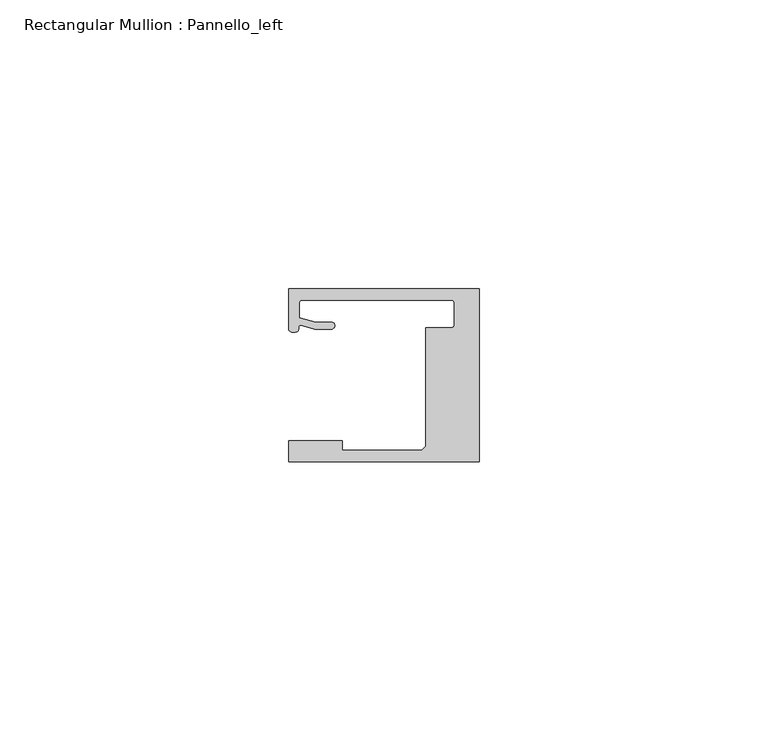
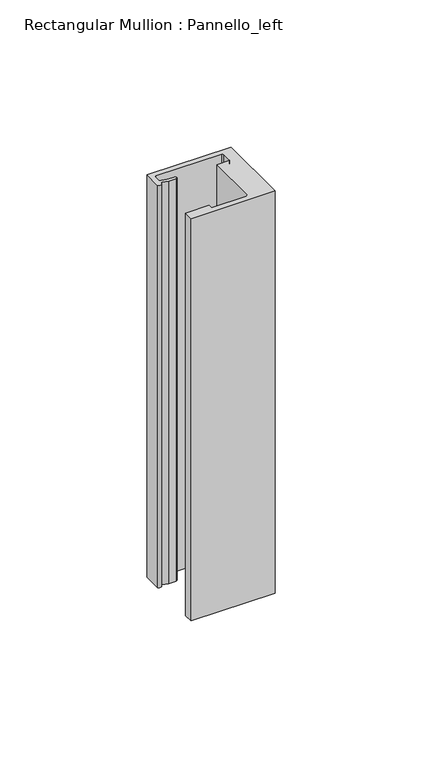
"""IFC4 building model written with IfcOpenShell, lengths in millimetres: member geometry, Rectangular Mullion : Pannello_left."""

from ifc_helpers import new_model, si_unit, frame, origin, place, context, project, spatial, polyline, circle_curve, source, transform, mapped, element, save
from ifc_brep_helpers import plane_surface, cylinder_surface, revolved_surface, extruded_surface, spline_curve, advanced_brep


def rectangular_mullion_pannello_left_600754f7(model_context):
    return source(origin(), model_context, "Body", "AdvancedBrep", [
        advanced_brep(
        [(-33.0, -15.0, 0.0), (0.0, -15.0, 0.0), (0.0, 15.0, 0.0), (-33.0000135, 15.0, 0.0), (-33.0000135, 8.0000472, 0.0), (-30.9223017, 8.6490241, 0.0), (-28.4999305, 7.9999523, 0.0), (-25.59998, 7.9999523, 0.0), (-25.59998, 9.1999523, 0.0), (-28.3419477, 9.1999523, 0.0), (-31.19998, 9.9657591, 0.0), (-31.19998, 12.50001, 0.0), (-30.69998, 13.00001, 0.0), (-4.7999726, 13.00001, 0.0), (-4.2999726, 12.50001, 0.0), (-4.2999726, 8.7500595, 0.0), (-4.7999726, 8.2500595, 0.0), (-9.2999726, 8.2500595, 0.0), (-9.2999726, -12.2999849, 0.0), (-10.0000103, -13.0000004, 0.0), (-23.700041, -13.0000004, 0.0), (-23.700041, -11.3000004, 0.0), (-33.0, -11.3000004, 0.0), (-33.0, -15.0, -166.9999865), (-33.0, -11.3000004, -166.9999865), (-23.700041, -11.3000004, -166.9999865), (-23.700041, -13.0000004, -166.9999865), (-10.0000103, -13.0000004, -166.9999865), (-9.2999726, -12.2999849, -166.9999865), (-9.2999726, 8.2500595, -166.9999865), (-4.7999726, 8.2500595, -166.9999865), (-4.2999726, 8.7500595, -166.9999865), (-4.2999726, 12.50001, -166.9999865), (-4.7999726, 13.00001, -166.9999865), (-30.69998, 13.00001, -166.9999865), (-31.19998, 12.50001, -166.9999865), (-31.19998, 9.9657591, -166.9999865), (-28.3419477, 9.1999523, -166.9999865), (-25.59998, 9.1999523, -166.9999865), (-25.59998, 7.9999523, -166.9999865), (-28.4999305, 7.9999523, -166.9999865), (-30.9223017, 8.6490241, -166.9999865), (-33.0000135, 8.0000472, -166.9999865), (-33.0000135, 15.0, -166.9999865), (0.0, 15.0, -166.9999865), (0.0, -15.0, -166.9999865)],
        [
            (0, 1),
            (1, 2),
            (2, 3),
            (3, 4),
            (4, 5, spline_curve(3, [(-33.0000135, 8.0000472, 0.0), (-33.0000135, 7.457047519, 0.0), (-32.262327879, 7.456527435, 0.0), (-31.357433266, 7.563996614, 0.0), (-31.305645054, 7.690065204, 0.0), (-31.298563602, 8.366228555, 0.0), (-31.312054066, 8.717747958, 0.0), (-30.9223017, 8.6490241, 0.0)], [4, 2, 2, 4], [0.0, 0.0027053965905959043, 0.0058611956533709, 0.007702013405570312])),
            (5, 6),
            (6, 7),
            (7, 8, circle_curve(frame((-25.59998, 8.5999523, 0.0), z_axis=(0.0, 0.0, 1.0), x_axis=(0.0, 1.0, 0.0)), 0.6)),
            (8, 9),
            (9, 10),
            (10, 11),
            (11, 12, circle_curve(frame((-30.69998, 12.50001, 0.0), z_axis=(0.0, 0.0, -1.0), x_axis=(0.0, 1.0, 0.0)), 0.5)),
            (12, 13),
            (13, 14, circle_curve(frame((-4.7999726, 12.50001, 0.0), z_axis=(0.0, 0.0, -1.0), x_axis=(1.0, 0.0, 0.0)), 0.5)),
            (14, 15),
            (15, 16, circle_curve(frame((-4.7999726, 8.7500595, 0.0), z_axis=(0.0, 0.0, -1.0), x_axis=(0.0, -1.0, 0.0)), 0.5)),
            (16, 17),
            (17, 18),
            (18, 19),
            (19, 20),
            (20, 21),
            (21, 22),
            (22, 0),
            (23, 24),
            (24, 25),
            (25, 26),
            (26, 27),
            (27, 28),
            (28, 29),
            (29, 30),
            (30, 31, circle_curve(frame((-4.7999726, 8.7500595, -166.9999865), z_axis=(0.0, 0.0, 1.0), x_axis=(0.0, -1.0, 0.0)), 0.5)),
            (31, 32),
            (32, 33, circle_curve(frame((-4.7999726, 12.50001, -166.9999865), z_axis=(0.0, 0.0, 1.0), x_axis=(1.0, 0.0, 0.0)), 0.5)),
            (33, 34),
            (34, 35, circle_curve(frame((-30.69998, 12.50001, -166.9999865), z_axis=(0.0, 0.0, 1.0), x_axis=(0.0, 1.0, 0.0)), 0.5)),
            (35, 36),
            (36, 37),
            (37, 38),
            (38, 39, circle_curve(frame((-25.59998, 8.5999523, -166.9999865), z_axis=(0.0, 0.0, -1.0), x_axis=(0.0, 1.0, 0.0)), 0.6)),
            (39, 40),
            (40, 41),
            (41, 42, spline_curve(3, [(-30.9223017, 8.6490241, -166.9999865), (-31.312054066, 8.717747958, -166.9999865), (-31.298563602, 8.366228555, -166.9999865), (-31.305645054, 7.690065204, -166.9999865), (-31.357433266, 7.563996614, -166.9999865), (-32.262327879, 7.456527435, -166.9999865), (-33.0000135, 7.457047519, -166.9999865), (-33.0000135, 8.0000472, -166.9999865)], [4, 2, 2, 4], [0.0, 0.001840817752199412, 0.004996616814974408, 0.007702013405570312])),
            (42, 43),
            (43, 44),
            (44, 45),
            (45, 23),
            (0, 23),
            (45, 1),
            (44, 2),
            (43, 3),
            (42, 4),
            (41, 5),
            (40, 6),
            (39, 7),
            (38, 8),
            (37, 9),
            (36, 10),
            (35, 11),
            (34, 12),
            (33, 13),
            (32, 14),
            (31, 15),
            (30, 16),
            (29, 17),
            (28, 18),
            (27, 19),
            (26, 20),
            (25, 21),
            (24, 22),
        ],
        [
            plane_surface(frame((0.0, -36.2491502, 0.0), z_axis=(0.0, 0.0, 1.0), x_axis=(-1.0, 0.0, 0.0))),
            plane_surface(frame((0.0, -36.2491502, -166.9999865), z_axis=(0.0, 0.0, -1.0), x_axis=(-1.0, 0.0, 0.0))),
            plane_surface(frame((-33.0, -15.0, 0.0), z_axis=(0.0, -1.0, 0.0), x_axis=(0.0, 0.0, -1.0))),
            plane_surface(frame((0.0, -15.0, 0.0), z_axis=(1.0, 0.0, 0.0), x_axis=(0.0, 0.0, -1.0))),
            plane_surface(frame((0.0, 15.0, 0.0), z_axis=(0.0, 1.0, 0.0), x_axis=(0.0, 0.0, -1.0))),
            plane_surface(frame((-33.0000135, 15.0, 0.0), z_axis=(-1.0, 0.0, 0.0), x_axis=(0.0, 0.0, -1.0))),
            extruded_surface(spline_curve(3, [(-33.0000135, 8.0000472, -166.9999865), (-33.0000135, 7.457047519, -166.9999865), (-32.262327879, 7.456527435, -166.9999865), (-31.357433266, 7.563996614, -166.9999865), (-31.305645054, 7.690065204, -166.9999865), (-31.298563602, 8.366228555, -166.9999865), (-31.312054066, 8.717747958, -166.9999865), (-30.9223017, 8.6490241, -166.9999865)], [4, 2, 2, 4], [0.0, 0.0027053965905959043, 0.0058611956533709, 0.007702013405570312]), (0.0, 0.0, 166.9999865), 166.9999865),
            plane_surface(frame((-30.9223017, 8.6490241, 0.0), z_axis=(-0.25881883200192934, -0.9659258833891746, 0.0), x_axis=(0.0, 0.0, -1.0))),
            plane_surface(frame((-28.4999305, 7.9999523, 0.0), z_axis=(0.0, -1.0, 0.0), x_axis=(0.0, 0.0, -1.0))),
            cylinder_surface(frame((-25.59998, 8.5999523, 0.0), z_axis=(0.0, 0.0, 1.0), x_axis=(0.0, 1.0, 0.0)), 0.6),
            plane_surface(frame((-25.59998, 9.1999523, 0.0), z_axis=(0.0, 1.0, 0.0), x_axis=(0.0, 0.0, -1.0))),
            plane_surface(frame((-28.3419477, 9.1999523, 0.0), z_axis=(0.25881883204288636, 0.9659258833782002, 0.0), x_axis=(0.0, 0.0, -1.0))),
            plane_surface(frame((-31.19998, 9.9657591, 0.0), z_axis=(1.0, 0.0, 0.0), x_axis=(0.0, 0.0, -1.0))),
            revolved_surface(polyline([(-30.69998, 13.00001, -166.9999865), (-30.69998, 13.00001, 0.0)]), (-30.69998, 12.50001, 0.0), (0.0, 0.0, -1.0)),
            plane_surface(frame((-30.69998, 13.00001, 0.0), z_axis=(0.0, -1.0, 0.0), x_axis=(0.0, 0.0, -1.0))),
            revolved_surface(polyline([(-4.2999726, 12.50001, -166.9999865), (-4.2999726, 12.50001, 0.0)]), (-4.7999726, 12.50001, 0.0), (0.0, 0.0, -1.0)),
            plane_surface(frame((-4.2999726, 12.50001, 0.0), z_axis=(-1.0, 0.0, 0.0), x_axis=(0.0, 0.0, -1.0))),
            revolved_surface(polyline([(-4.7999726, 8.2500595, -166.9999865), (-4.7999726, 8.2500595, 0.0)]), (-4.7999726, 8.7500595, 0.0), (0.0, 0.0, -1.0)),
            plane_surface(frame((-4.7999726, 8.2500595, 0.0), z_axis=(0.0, 1.0, 0.0), x_axis=(0.0, 0.0, -1.0))),
            plane_surface(frame((-9.2999726, 8.2500595, 0.0), z_axis=(-1.0, 0.0, 0.0), x_axis=(0.0, 0.0, -1.0))),
            plane_surface(frame((-9.2999726, -12.2999849, 0.0), z_axis=(-0.7070955486277984, 0.7071180135668678, 0.0), x_axis=(0.0, 0.0, -1.0))),
            plane_surface(frame((-10.0000103, -13.0000004, 0.0), z_axis=(0.0, 1.0, 0.0), x_axis=(0.0, 0.0, -1.0))),
            plane_surface(frame((-23.700041, -13.0000004, 0.0), z_axis=(1.0, 0.0, 0.0), x_axis=(0.0, 0.0, -1.0))),
            plane_surface(frame((-23.700041, -11.3000004, 0.0), z_axis=(0.0, 1.0, 0.0), x_axis=(0.0, 0.0, -1.0))),
            plane_surface(frame((-33.0, -11.3000004, 0.0), z_axis=(-1.0, 0.0, 0.0), x_axis=(0.0, 0.0, -1.0))),
        ],
        [
            (0, [[1, 2, 3, 4, 5, 6, 7, 8, 9, 10, 11, 12, 13, 14, 15, 16, 17, 18, 19, 20, 21, 22, 23]]),
            (1, [[24, 25, 26, 27, 28, 29, 30, 31, 32, 33, 34, 35, 36, 37, 38, 39, 40, 41, 42, 43, 44, 45, 46]]),
            (2, [[-1, 47, -46, 48]]),
            (3, [[-2, -48, -45, 49]]),
            (4, [[-3, -49, -44, 50]]),
            (5, [[-4, -50, -43, 51]]),
            (6, [[-5, -51, -42, 52]]),
            (7, [[-6, -52, -41, 53]]),
            (8, [[-7, -53, -40, 54]]),
            (9, [[-8, -54, -39, 55]]),
            (10, [[-9, -55, -38, 56]]),
            (11, [[-10, -56, -37, 57]]),
            (12, [[-11, -57, -36, 58]]),
            (13, [[-12, -58, -35, 59]]),
            (14, [[-13, -59, -34, 60]]),
            (15, [[-14, -60, -33, 61]]),
            (16, [[-15, -61, -32, 62]]),
            (17, [[-16, -62, -31, 63]]),
            (18, [[-17, -63, -30, 64]]),
            (19, [[-18, -64, -29, 65]]),
            (20, [[-19, -65, -28, 66]]),
            (21, [[-20, -66, -27, 67]]),
            (22, [[-21, -67, -26, 68]]),
            (23, [[-22, -68, -25, 69]]),
            (24, [[-23, -69, -24, -47]]),
        ],
    ),
    ])


if __name__ == "__main__":
    model = new_model("IFC4")
    model_context = context("Model", 3, world=origin())
    ifc_project = project(units=[si_unit("LENGTHUNIT", "METRE", prefix="MILLI")], contexts=[model_context])
    site = spatial("IfcSite", under=ifc_project)
    building = spatial("IfcBuilding", under=site)
    placement = place(None, origin())
    rectangular_mullion_pannello_left_shape = rectangular_mullion_pannello_left_600754f7(model_context)
    element("IfcMember", 1, ObjectType="Rectangular Mullion : Pannello_left", at=placement, inside=building, context=model_context, shape_type="MappedRepresentation", body=[
        mapped(rectangular_mullion_pannello_left_shape, transform((0.0, 0.0, 0.0), x_axis=(1.0, 0.0, 0.0), y_axis=(0.0, 1.0, 0.0), z_axis=(0.0, 0.0, 1.0))),
    ])
    save(model, "model.ifc")

# Revit data of these elements
# Type "Rectangular Mullion : Pannello_left"
#   built-in parameter 1007322 = 0.0984252 (stored number, unit not read)
#   built-in parameter 1007320 = 0.0305117 (stored number, unit not read)
